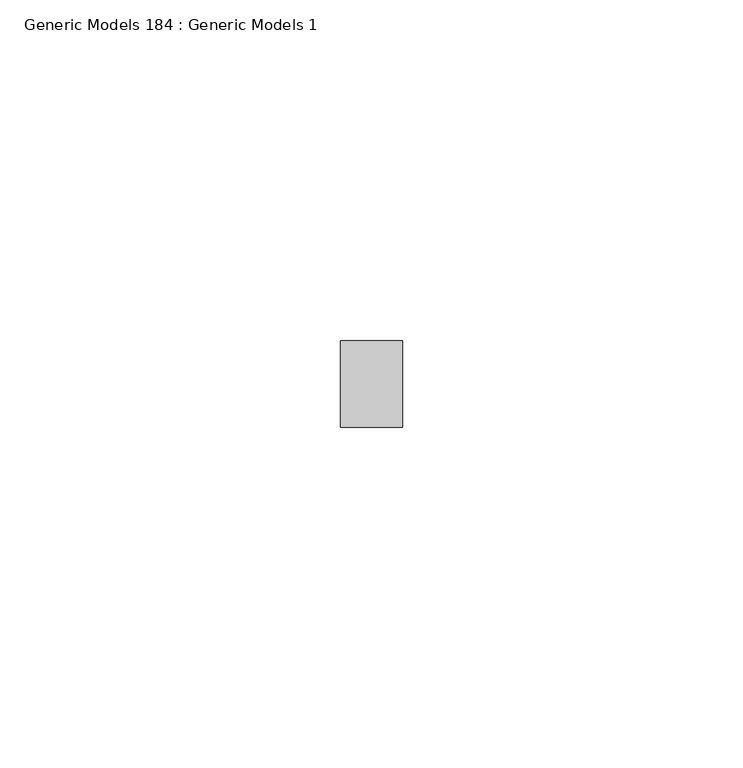
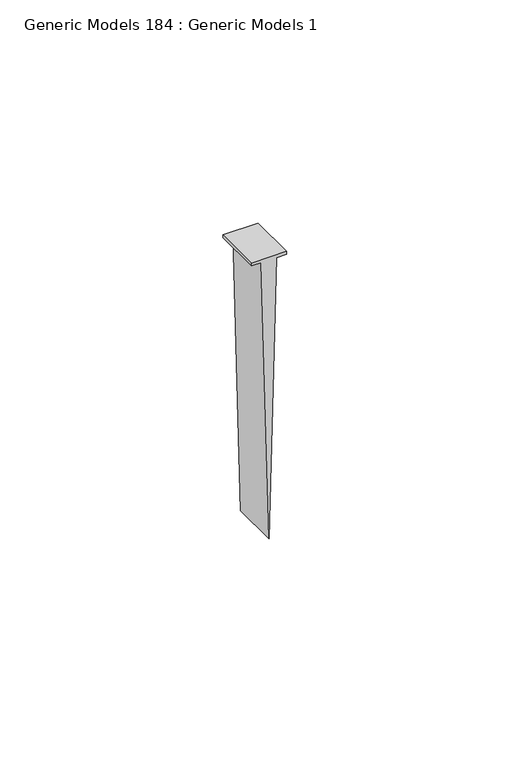
"""IFC4 building model written with IfcOpenShell, lengths in millimetres: proxy geometry, Generic Models 184 : Generic Models 1."""

from ifc_helpers import new_model, si_unit, frame, origin, place, context, project, spatial, polyline, outline, extrude, source, transform, mapped, element, save


def generic_models_184_generic_models_1_43150da2(model_context):
    return source(origin(), model_context, "Body", "SweptSolid", [
        extrude(outline(polyline([(39.6875, 48511.0409), (38.89375, 48511.0409), (38.89375, 48513.5907636), (-37.30625, 48515.5875), (38.89375, 48517.5842364), (38.89375, 48520.1341), (39.6875, 48520.1341), (39.6875, 48511.0409)])), frame((0.0, 565.15, 0.0), z_axis=(0.0, 1.0, 0.0), x_axis=(0.0, 0.0, 1.0)), (0.0, 0.0, 1.0), 12.7),
    ])


if __name__ == "__main__":
    model = new_model("IFC4")
    model_context = context("Model", 3, world=origin())
    ifc_project = project(units=[si_unit("LENGTHUNIT", "METRE", prefix="MILLI")], contexts=[model_context])
    site = spatial("IfcSite", under=ifc_project)
    building = spatial("IfcBuilding", under=site)
    placement = place(None, origin())
    generic_models_184_generic_models_1_shape = generic_models_184_generic_models_1_43150da2(model_context)
    element("IfcBuildingElementProxy", 1, Name="Generic Models 184 : Generic Models 1", ObjectType="Generic Models 184 : Generic Models 1", at=placement, inside=building, context=model_context, shape_type="MappedRepresentation", body=[
        mapped(generic_models_184_generic_models_1_shape, transform((0.0, 0.0, 0.0), x_axis=(1.0, 0.0, 0.0), y_axis=(0.0, 1.0, 0.0), z_axis=(0.0, 0.0, 1.0))),
    ])
    save(model, "model.ifc")

# Revit data of these elements
# Element 1 (IfcBuildingElementProxy, "Generic Models 184 : Generic Models 1")
#   Materials on its faces: "ATTACH GYPSUM BOARD TO STUDS AND NOT TO TOP TRACK"
# Materials
#   "ATTACH GYPSUM BOARD TO STUDS AND NOT TO TOP TRACK": class "Generic", colour RGB 48 48 48, transparency 0, Cost = 0
